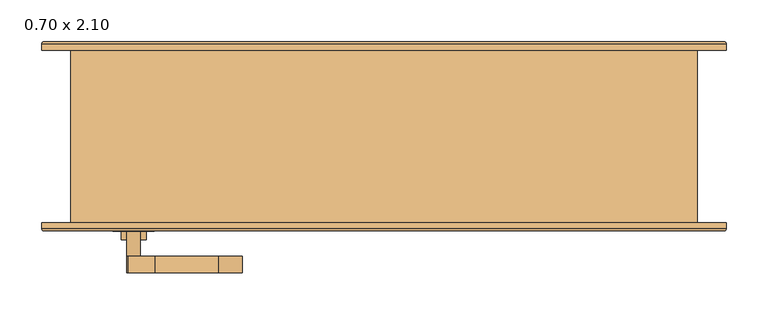
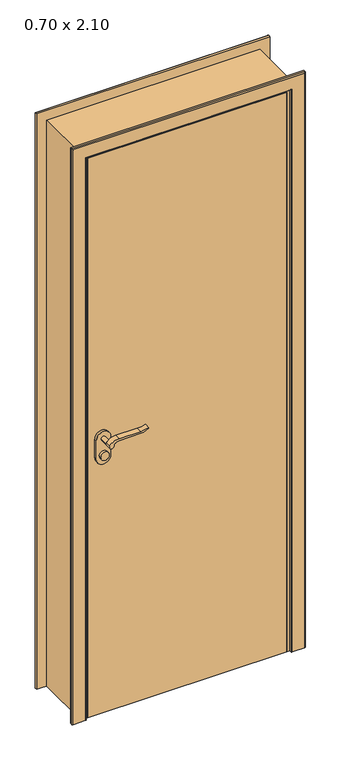
"""IFC4 building model written with IfcOpenShell, lengths in millimetres: door geometry, .CC_ND 300_PORTA SIMPLES DE ABRIR_COM EXTENSÃO : 0.70 x 2.10."""

from ifc_helpers import new_model, si_unit, point, frame, frame_2d, origin, origin_with_axes, place, context, project, spatial, polyline, circle_curve, ellipse_curve, trimmed, segment, composite_curve, outline, extrude, faceted_brep, source, transform, mapped, element, save
from ifc_brep_helpers import plane_surface, cylinder_surface, advanced_brep


def door_0_70_x_2_10_2730a6bb(model_context):
    return source(origin(), model_context, "Body", "SolidModel", [
        extrude(outline(composite_curve([segment(trimmed(circle_curve(frame_2d((964.5, -300.0)), 15.0), [point((964.5, -285.0))], [point((964.5, -315.0))], False, "CARTESIAN"), True, "CONTINUOUS"), segment(trimmed(circle_curve(frame_2d((964.5, -300.0)), 15.0), [point((964.5, -315.0))], [point((964.5, -285.0))], False, "CARTESIAN"), True, "CONTINUOUS")], self_intersect=False)), frame((0.0, -120.7, 0.0), z_axis=(0.0, 1.0, 0.0), x_axis=(0.0, 0.0, 1.0)), (0.0, 0.0, 1.0), 10.0),
        extrude(outline(composite_curve([segment(trimmed(circle_curve(frame_2d((964.5, -300.0)), 15.0), [point((964.5, -285.0))], [point((964.5, -315.0))], False, "CARTESIAN"), True, "CONTINUOUS"), segment(trimmed(circle_curve(frame_2d((964.5, -300.0)), 15.0), [point((964.5, -315.0))], [point((964.5, -285.0))], False, "CARTESIAN"), True, "CONTINUOUS")], self_intersect=False)), frame((0.0, -60.7, 0.0), z_axis=(0.0, 1.0, 0.0), x_axis=(0.0, 0.0, 1.0)), (0.0, 0.0, 1.0), 10.0),
        extrude(outline(composite_curve([segment(trimmed(circle_curve(frame_2d((1024.5, -300.0)), 8.0), [point((1029.1523287, -306.5081363))], [point((1024.5, -292.0))], False, "CARTESIAN"), True, "CONTINUOUS"), segment(trimmed(circle_curve(frame_2d((1019.3738613, -274.6138099)), 18.1261387), [point((1024.5, -292.0))], [point((1037.5, -274.6138099))], True, "CARTESIAN"), True, "CONTINUOUS"), segment(polyline([(1037.5, -274.6138099), (1037.5, -198.3564091)]), True, "CONTINUOUS"), segment(trimmed(circle_curve(frame_2d((1096.7709207, -201.9396612)), 59.3791355), [point((1037.5, -198.3564091))], [point((1046.7135558, -170.0))], False, "CARTESIAN"), True, "CONTINUOUS"), segment(polyline([(1046.7135558, -170.0), (1049.5, -170.0)]), True, "CONTINUOUS"), segment(trimmed(circle_curve(frame_2d((1127.7850638, -198.4227909)), 83.2850902), [point((1049.5, -170.0))], [point((1044.5, -198.3564091))], True, "CARTESIAN"), True, "CONTINUOUS"), segment(polyline([(1044.5, -198.3564091), (1044.5, -274.6325667)]), True, "CONTINUOUS"), segment(trimmed(circle_curve(frame_2d((1007.2555521, -276.3324871)), 37.2832219), [point((1044.5, -274.6325667))], [point((1029.1523287, -306.5081363))], False, "CARTESIAN"), True, "CONTINUOUS")], self_intersect=False)), frame((0.0, -160.7, 0.0), z_axis=(0.0, 1.0, 0.0), x_axis=(0.0, 0.0, 1.0)), (0.0, 0.0, 1.0), 20.0),
        extrude(outline(composite_curve([segment(trimmed(circle_curve(frame_2d((1019.3738682, -274.6138122)), 18.1261318), [point((1024.4999903, -292.0))], [point((1037.5, -274.6138122))], True, "CARTESIAN"), True, "CONTINUOUS"), segment(polyline([(1037.5, -274.6138122), (1037.5, -198.3564091)]), True, "CONTINUOUS"), segment(trimmed(circle_curve(frame_2d((1096.7709207, -201.9396612)), 59.3791355), [point((1037.5, -198.3564091))], [point((1046.7135558, -170.0))], False, "CARTESIAN"), True, "CONTINUOUS"), segment(polyline([(1046.7135558, -170.0), (1049.5, -170.0)]), True, "CONTINUOUS"), segment(trimmed(circle_curve(frame_2d((1127.7850638, -198.4227909)), 83.2850902), [point((1049.5, -170.0))], [point((1044.5, -198.3564091))], True, "CARTESIAN"), True, "CONTINUOUS"), segment(polyline([(1044.5, -198.3564091), (1044.5, -274.6325667)]), True, "CONTINUOUS"), segment(trimmed(circle_curve(frame_2d((1007.2555521, -276.3324871)), 37.2832219), [point((1044.5, -274.6325667))], [point((1029.1523287, -306.5081363))], False, "CARTESIAN"), True, "CONTINUOUS"), segment(trimmed(circle_curve(frame_2d((1024.5, -300.0)), 8.0), [point((1029.1523287, -306.5081363))], [point((1024.4999903, -292.0))], False, "CARTESIAN"), True, "CONTINUOUS")], self_intersect=False)), frame((0.0, -30.7, 0.0), z_axis=(0.0, 1.0, 0.0), x_axis=(0.0, 0.0, 1.0)), (0.0, 0.0, 1.0), 20.0),
        extrude(outline(composite_curve([segment(trimmed(circle_curve(frame_2d((1024.5, -300.0)), 8.0), [point((1024.5, -292.0))], [point((1024.5, -308.0))], False, "CARTESIAN"), True, "CONTINUOUS"), segment(trimmed(circle_curve(frame_2d((1024.5, -300.0)), 8.0), [point((1024.5, -308.0))], [point((1024.5, -292.0))], False, "CARTESIAN"), True, "CONTINUOUS")], self_intersect=False)), frame((0.0, -140.7, 0.0), z_axis=(0.0, 1.0, 0.0), x_axis=(0.0, 0.0, 1.0)), (0.0, 0.0, 1.0), 30.0),
        extrude(outline(composite_curve([segment(trimmed(circle_curve(frame_2d((1024.5, -300.0)), 8.0), [point((1024.5, -292.0))], [point((1024.5, -308.0))], False, "CARTESIAN"), True, "CONTINUOUS"), segment(trimmed(circle_curve(frame_2d((1024.5, -300.0)), 8.0), [point((1024.5, -308.0))], [point((1024.5, -292.0))], False, "CARTESIAN"), True, "CONTINUOUS")], self_intersect=False)), frame((0.0, -60.7, 0.0), z_axis=(0.0, 1.0, 0.0), x_axis=(0.0, 0.0, 1.0)), (0.0, 0.0, 1.0), 30.0),
        extrude(outline(composite_curve([segment(trimmed(circle_curve(frame_2d((954.5, -300.0)), 25.0), [point((954.5, -325.0))], [point((954.5, -275.0))], False, "CARTESIAN"), True, "CONTINUOUS"), segment(polyline([(954.5, -275.0), (1024.5, -275.0)]), True, "CONTINUOUS"), segment(trimmed(circle_curve(frame_2d((1024.5, -300.0)), 25.0), [point((1024.5, -275.0))], [point((1024.5, -325.0))], False, "CARTESIAN"), True, "CONTINUOUS"), segment(polyline([(1024.5, -325.0), (954.5, -325.0)]), True, "CONTINUOUS")], self_intersect=False)), frame((0.0, -110.7, 0.0), z_axis=(0.0, 1.0, 0.0), x_axis=(0.0, 0.0, 1.0)), (0.0, 0.0, 1.0), 10.0),
        extrude(outline(composite_curve([segment(trimmed(circle_curve(frame_2d((954.5, -300.0)), 25.0), [point((954.5, -325.0))], [point((954.5, -275.0))], False, "CARTESIAN"), True, "CONTINUOUS"), segment(polyline([(954.5, -275.0), (1024.5, -275.0)]), True, "CONTINUOUS"), segment(trimmed(circle_curve(frame_2d((1024.5, -300.0)), 25.0), [point((1024.5, -275.0))], [point((1024.5, -325.0))], False, "CARTESIAN"), True, "CONTINUOUS"), segment(polyline([(1024.5, -325.0), (954.5, -325.0)]), True, "CONTINUOUS")], self_intersect=False)), frame((0.0, -70.7, 0.0), z_axis=(0.0, 1.0, 0.0), x_axis=(0.0, 0.0, 1.0)), (0.0, 0.0, 1.0), 10.0),
        faceted_brep([(342.0, 106.0, 0.0), (375.0, 106.0, 0.0), (375.0, -100.7, 0.0), (350.0, -100.7, 0.0), (350.0, -70.7, 0.0), (342.0, -70.7, 0.0), (342.0, 106.0, 2067.0), (-342.0, 106.0, 2067.0), (-342.0, 106.0, 0.0), (-375.0, 106.0, 0.0), (-375.0, 106.0, 2100.0), (375.0, 106.0, 2100.0), (375.0, -100.7, 2100.0), (-375.0, -100.7, 2100.0), (-375.0, -100.7, 0.0), (-350.0, -100.7, 0.0), (-350.0, -100.7, 2075.0), (350.0, -100.7, 2075.0), (350.0, -70.7, 2075.0), (-350.0, -70.7, 2075.0), (-350.0, -70.7, 0.0), (-342.0, -70.7, 0.0), (-342.0, -70.7, 2067.0), (342.0, -70.7, 2067.0)], [[[0, 1, 2, 3, 4, 5]], [[1, 0, 6, 7, 8, 9, 10, 11]], [[2, 1, 11, 12]], [[3, 2, 12, 13, 14, 15, 16, 17]], [[4, 3, 17, 18]], [[5, 4, 18, 19, 20, 21, 22, 23]], [[0, 5, 23, 6]], [[7, 22, 21, 8]], [[8, 21, 20, 15, 14, 9]], [[13, 10, 9, 14]], [[19, 16, 15, 20]], [[12, 11, 10, 13]], [[18, 17, 16, 19]], [[6, 23, 22, 7]]]),
        extrude(outline(polyline([(-350.0, -70.7), (350.0, -70.7), (350.0, -100.7), (-350.0, -100.7), (-350.0, -70.7)])), origin_with_axes(), (0.0, 0.0, 1.0), 2075.0),
        advanced_brep(
        [(-410.0, -100.7, 0.0), (-360.0, -100.7, 0.0), (-360.0, -107.7, 0.0), (-363.0, -110.7, 0.0), (-407.0, -110.7, 0.0), (-410.0, -107.7, 0.0), (-410.0, -100.7, 2135.0), (410.0, -100.7, 2135.0), (410.0, -100.7, 0.0), (360.0, -100.7, 0.0), (360.0, -100.7, 2085.0), (-360.0, -100.7, 2085.0), (-360.0, -107.7, 2085.0), (-363.0, -110.7, 2088.0), (363.0, -110.7, 2088.0), (363.0, -110.7, 0.0), (407.0, -110.7, 0.0), (407.0, -110.7, 2132.0), (-407.0, -110.7, 2132.0), (-410.0, -107.7, 2135.0), (410.0, -107.7, 2135.0), (410.0, -107.7, 0.0), (360.0, -107.7, 0.0), (360.0, -107.7, 2085.0)],
        [
            (0, 1),
            (1, 2),
            (2, 3, circle_curve(frame((-363.0, -107.7, 0.0), z_axis=(0.0, 0.0, -1.0), x_axis=(1.0, 0.0, 0.0)), 3.0)),
            (3, 4),
            (4, 5, circle_curve(frame((-407.0, -107.7, 0.0), z_axis=(0.0, 0.0, -1.0), x_axis=(1.0, 0.0, 0.0)), 3.0)),
            (5, 0),
            (0, 6),
            (6, 7),
            (7, 8),
            (8, 9),
            (9, 10),
            (10, 11),
            (11, 1),
            (11, 12),
            (12, 2),
            (12, 13, ellipse_curve(frame((-363.0, -107.7, 2088.0), z_axis=(-0.7071067811865475, 0.0, -0.7071067811865475), x_axis=(0.7071067811865474, 0.0, -0.7071067811865476)), 4.2426407, 3.0)),
            (13, 3),
            (13, 14),
            (14, 15),
            (15, 16),
            (16, 17),
            (17, 18),
            (18, 4),
            (18, 19, ellipse_curve(frame((-407.0, -107.7, 2132.0), z_axis=(-0.7071067811865475, 0.0, -0.7071067811865475), x_axis=(0.7071067811865474, 0.0, -0.7071067811865476)), 4.2426407, 3.0)),
            (19, 5),
            (19, 6),
            (7, 20),
            (20, 21),
            (21, 8),
            (21, 16, circle_curve(frame((407.0, -107.7, 0.0), z_axis=(0.0, 0.0, -1.0), x_axis=(-1.0, 0.0, 0.0)), 3.0)),
            (15, 22, circle_curve(frame((363.0, -107.7, 0.0), z_axis=(0.0, 0.0, -1.0), x_axis=(-1.0, 0.0, 0.0)), 3.0)),
            (22, 9),
            (23, 10),
            (22, 23),
            (14, 23, ellipse_curve(frame((363.0, -107.7, 2088.0), z_axis=(0.7071067811865475, 0.0, -0.7071067811865475), x_axis=(0.7071067811865474, 0.0, 0.7071067811865476)), 4.2426407, 3.0)),
            (20, 17, ellipse_curve(frame((407.0, -107.7, 2132.0), z_axis=(0.7071067811865475, 0.0, -0.7071067811865475), x_axis=(0.7071067811865474, 0.0, 0.7071067811865476)), 4.2426407, 3.0)),
            (23, 12),
            (19, 20),
        ],
        [
            plane_surface(frame((-360.0, -100.7, 0.0), z_axis=(0.0, 0.0, -1.0), x_axis=(0.0, 1.0, 0.0))),
            plane_surface(frame((-410.0, -100.7, 0.0), z_axis=(0.0, 1.0, 0.0), x_axis=(0.0, 0.0, 1.0))),
            plane_surface(frame((-360.0, -100.7, 0.0), z_axis=(1.0, 0.0, 0.0), x_axis=(0.0, 0.0, 1.0))),
            cylinder_surface(frame((-363.0, -107.7, 0.0), z_axis=(0.0, 0.0, -1.0), x_axis=(1.0, 0.0, 0.0)), 3.0),
            plane_surface(frame((-363.0, -110.7, 0.0), z_axis=(0.0, -1.0, 0.0), x_axis=(0.0, 0.0, 1.0))),
            cylinder_surface(frame((-407.0, -107.7, 0.0), z_axis=(0.0, 0.0, -1.0), x_axis=(1.0, 0.0, 0.0)), 3.0),
            plane_surface(frame((-410.0, -107.7, 0.0), z_axis=(-1.0, 0.0, 0.0), x_axis=(0.0, 0.0, 1.0))),
            plane_surface(frame((410.0, -107.7, 2135.0), z_axis=(1.0, 0.0, 0.0), x_axis=(0.0, 0.0, -1.0))),
            plane_surface(frame((360.0, -100.7, 0.0), z_axis=(0.0, 0.0, -1.0), x_axis=(0.0, 1.0, 0.0))),
            plane_surface(frame((360.0, -100.7, 2085.0), z_axis=(-1.0, 0.0, 0.0), x_axis=(0.0, 0.0, -1.0))),
            cylinder_surface(frame((363.0, -107.7, 2085.0), z_axis=(0.0, 0.0, 1.0), x_axis=(-1.0, 0.0, 0.0)), 3.0),
            cylinder_surface(frame((407.0, -107.7, 2085.0), z_axis=(0.0, 0.0, 1.0), x_axis=(-1.0, 0.0, 0.0)), 3.0),
            plane_surface(frame((-360.0, -100.7, 2085.0), z_axis=(0.0, 0.0, -1.0), x_axis=(1.0, 0.0, 0.0))),
            plane_surface(frame((-410.0, -107.7, 2135.0), z_axis=(0.0, 0.0, 1.0), x_axis=(1.0, 0.0, 0.0))),
            cylinder_surface(frame((-360.0, -107.7, 2088.0), z_axis=(-1.0, 0.0, 0.0), x_axis=(0.0, 0.0, -1.0)), 3.0),
            cylinder_surface(frame((-360.0, -107.7, 2132.0), z_axis=(-1.0, 0.0, 0.0), x_axis=(0.0, 0.0, -1.0)), 3.0),
        ],
        [
            (0, [[1, 2, 3, 4, 5, 6]]),
            (1, [[-1, 7, 8, 9, 10, 11, 12, 13]]),
            (2, [[-2, -13, 14, 15]]),
            (3, [[-3, -15, 16, 17]]),
            (4, [[-4, -17, 18, 19, 20, 21, 22, 23]]),
            (5, [[-5, -23, 24, 25]]),
            (6, [[-6, -25, 26, -7]]),
            (7, [[27, 28, 29, -9]]),
            (8, [[-29, 30, -20, 31, 32, -10]]),
            (9, [[33, -11, -32, 34]]),
            (10, [[35, -34, -31, -19]]),
            (11, [[36, -21, -30, -28]]),
            (12, [[-14, -12, -33, 37]]),
            (13, [[-26, 38, -27, -8]]),
            (14, [[-16, -37, -35, -18]]),
            (15, [[-24, -22, -36, -38]]),
        ],
    ),
        advanced_brep(
        [(410.0, 106.0, 0.0), (360.0, 106.0, 0.0), (360.0, 113.0157283, 0.0), (362.9842717, 116.0, 0.0), (407.0342217, 116.0, 0.0), (410.0, 113.0342217, 0.0), (410.0, 106.0, 2135.0), (-410.0, 106.0, 2135.0), (-410.0, 106.0, 0.0), (-360.0, 106.0, 0.0), (-360.0, 106.0, 2085.0), (360.0, 106.0, 2085.0), (360.0, 113.0157283, 2085.0), (362.9842717, 116.0, 2087.9842717), (-362.9842717, 116.0, 2087.9842717), (-362.9842717, 116.0, 0.0), (-407.0342217, 116.0, 0.0), (-407.0342217, 116.0, 2132.0342217), (407.0342217, 116.0, 2132.0342217), (410.0, 113.0342217, 2135.0), (-410.0, 113.0342217, 2135.0), (-410.0, 113.0342217, 0.0), (-360.0, 113.0157283, 0.0), (-360.0, 113.0157283, 2085.0)],
        [
            (0, 1),
            (1, 2),
            (2, 3, circle_curve(frame((362.9842717, 113.0157283, 0.0), z_axis=(0.0, 0.0, -1.0), x_axis=(1.0, 0.0, 0.0)), 2.9842717)),
            (3, 4),
            (4, 5, circle_curve(frame((407.0342217, 113.0342217, 0.0), z_axis=(0.0, 0.0, -1.0), x_axis=(1.0, 0.0, 0.0)), 2.9657783)),
            (5, 0),
            (0, 6),
            (6, 7),
            (7, 8),
            (8, 9),
            (9, 10),
            (10, 11),
            (11, 1),
            (11, 12),
            (12, 2),
            (12, 13, ellipse_curve(frame((362.9842717, 113.0157283, 2087.9842717), z_axis=(0.7071067811865475, 0.0, -0.7071067811865475), x_axis=(-0.7071067811865474, 0.0, -0.7071067811865476)), 4.2203975, 2.9842717)),
            (13, 3),
            (13, 14),
            (14, 15),
            (15, 16),
            (16, 17),
            (17, 18),
            (18, 4),
            (18, 19, ellipse_curve(frame((407.0342217, 113.0342217, 2132.0342217), z_axis=(0.7071067811865475, 0.0, -0.7071067811865475), x_axis=(-0.7071067811865474, 0.0, -0.7071067811865476)), 4.1942438, 2.9657783)),
            (19, 5),
            (19, 6),
            (7, 20),
            (20, 21),
            (21, 8),
            (21, 16, circle_curve(frame((-407.0342217, 113.0342217, 0.0), z_axis=(0.0, 0.0, -1.0), x_axis=(-1.0, 0.0, 0.0)), 2.9657783)),
            (15, 22, circle_curve(frame((-362.9842717, 113.0157283, 0.0), z_axis=(0.0, 0.0, -1.0), x_axis=(-1.0, 0.0, 0.0)), 2.9842717)),
            (22, 9),
            (23, 10),
            (22, 23),
            (14, 23, ellipse_curve(frame((-362.9842717, 113.0157283, 2087.9842717), z_axis=(-0.7071067811865475, 0.0, -0.7071067811865475), x_axis=(-0.7071067811865474, 0.0, 0.7071067811865476)), 4.2203975, 2.9842717)),
            (20, 17, ellipse_curve(frame((-407.0342217, 113.0342217, 2132.0342217), z_axis=(-0.7071067811865475, 0.0, -0.7071067811865475), x_axis=(-0.7071067811865474, 0.0, 0.7071067811865476)), 4.1942438, 2.9657783)),
            (23, 12),
            (19, 20),
        ],
        [
            plane_surface(frame((360.0, 106.0, 0.0), z_axis=(0.0, 0.0, -1.0), x_axis=(0.0, 1.0, 0.0))),
            plane_surface(frame((410.0, 106.0, 0.0), z_axis=(0.0, -1.0, 0.0), x_axis=(0.0, 0.0, 1.0))),
            plane_surface(frame((360.0, 106.0, 0.0), z_axis=(-1.0, 0.0, 0.0), x_axis=(0.0, 0.0, 1.0))),
            cylinder_surface(frame((362.9842717, 113.0157283, 0.0), z_axis=(0.0, 0.0, -1.0), x_axis=(1.0, 0.0, 0.0)), 2.9842717),
            plane_surface(frame((362.9842717, 116.0, 0.0), z_axis=(0.0, 1.0, 0.0), x_axis=(0.0, 0.0, 1.0))),
            cylinder_surface(frame((407.0342217, 113.0342217, 0.0), z_axis=(0.0, 0.0, -1.0), x_axis=(1.0, 0.0, 0.0)), 2.9657783),
            plane_surface(frame((410.0, 113.0342217, 0.0), z_axis=(1.0, 0.0, 0.0), x_axis=(0.0, 0.0, 1.0))),
            plane_surface(frame((-410.0, 113.0342217, 2135.0), z_axis=(-1.0, 0.0, 0.0), x_axis=(0.0, 0.0, -1.0))),
            plane_surface(frame((-360.0, 106.0, 0.0), z_axis=(0.0, 0.0, -1.0), x_axis=(0.0, 1.0, 0.0))),
            plane_surface(frame((-360.0, 106.0, 2085.0), z_axis=(1.0, 0.0, 0.0), x_axis=(0.0, 0.0, -1.0))),
            cylinder_surface(frame((-362.9842717, 113.0157283, 2085.0), z_axis=(0.0, 0.0, 1.0), x_axis=(-1.0, 0.0, 0.0)), 2.9842717),
            cylinder_surface(frame((-407.0342217, 113.0342217, 2085.0), z_axis=(0.0, 0.0, 1.0), x_axis=(-1.0, 0.0, 0.0)), 2.9657783),
            plane_surface(frame((360.0, 106.0, 2085.0), z_axis=(0.0, 0.0, -1.0), x_axis=(-1.0, 0.0, 0.0))),
            plane_surface(frame((410.0, 113.0342217, 2135.0), z_axis=(0.0, 0.0, 1.0), x_axis=(-1.0, 0.0, 0.0))),
            cylinder_surface(frame((360.0, 113.0157283, 2087.9842717), z_axis=(1.0, 0.0, 0.0), x_axis=(0.0, 0.0, 1.0)), 2.9842717),
            cylinder_surface(frame((360.0, 113.0342217, 2132.0342217), z_axis=(1.0, 0.0, 0.0), x_axis=(0.0, 0.0, 1.0)), 2.9657783),
        ],
        [
            (0, [[1, 2, 3, 4, 5, 6]]),
            (1, [[-1, 7, 8, 9, 10, 11, 12, 13]]),
            (2, [[-2, -13, 14, 15]]),
            (3, [[-3, -15, 16, 17]]),
            (4, [[-4, -17, 18, 19, 20, 21, 22, 23]]),
            (5, [[-5, -23, 24, 25]]),
            (6, [[-6, -25, 26, -7]]),
            (7, [[27, 28, 29, -9]]),
            (8, [[-29, 30, -20, 31, 32, -10]]),
            (9, [[33, -11, -32, 34]]),
            (10, [[35, -34, -31, -19]]),
            (11, [[36, -21, -30, -28]]),
            (12, [[-14, -12, -33, 37]]),
            (13, [[-26, 38, -27, -8]]),
            (14, [[-16, -37, -35, -18]]),
            (15, [[-24, -22, -36, -38]]),
        ],
    ),
    ])


if __name__ == "__main__":
    model = new_model("IFC4")
    model_context = context("Model", 3, world=origin())
    ifc_project = project(units=[si_unit("LENGTHUNIT", "METRE", prefix="MILLI")], contexts=[model_context])
    site = spatial("IfcSite", under=ifc_project)
    building = spatial("IfcBuilding", under=site)
    placement = place(None, origin())
    door_0_70_x_2_10_shape = door_0_70_x_2_10_2730a6bb(model_context)
    element("IfcDoor", 1, ObjectType=".CC_ND 300_PORTA SIMPLES DE ABRIR_COM EXTENSÃO : 0.70 x 2.10", at=placement, inside=building, context=model_context, shape_type="MappedRepresentation", body=[
        mapped(door_0_70_x_2_10_shape, transform((0.0, 0.0, 0.0), x_axis=(1.0, 0.0, 0.0), y_axis=(0.0, 1.0, 0.0), z_axis=(0.0, 0.0, 1.0))),
    ])
    save(model, "model.ifc")

# Revit data of these elements
# Type ".CC_ND 300_PORTA SIMPLES DE ABRIR_COM EXTENSÃO : 0.70 x 2.10"
#   Type Mark = "155"
#   Analytic Construction = "<None>"
#   Rough Width = 0.75 m
#   Espessura moldura externa = 0.01 m
#   Espessura moldura interna = 0.01 m
#   Largura moldura = 0.05 m
#   Extensão acabamento exterior [instance default] = 0.00 m
#   Extensão acabamento interior [instance default] = 0.00 m
#   Espessura batente = 0.025 m
#   Thickness = 0.03 m
#   Altura batente = 2.085 m
#   Aux Arco [instance default] = 0.70 m
#   Rough Height = 2.125 m
#   Height = 2.10 m
#   Width = 0.70 m
#   Moldura interna [instance default] = yes
#   Moldura externa [instance default] = yes
#   Porta = .MADEIRA COM PINTURA ESMALTE BRANCO ACETINADO
#   Moldura = .MADEIRA COM PINTURA ESMALTE BRANCO ACETINADO
#   Maçaneta = .ALUMÍNIO
#   Batente = .MADEIRA COM PINTURA ESMALTE BRANCO ACETINADO
#   Function = (empty or 0)
#   Wall Closure = (empty or 0)
# Element 1 (IfcDoor, ".CC_ND 300_PORTA SIMPLES DE ABRIR_COM EXTENSÃO : 0.70 x 2.10")
#   Extensão acabamento exterior = 0.031 m
#   Extensão acabamento interior = 0.0257 m
#   Aux Arco = 0.7257 m
#   Materials on its faces: ".MADEIRA COM PINTURA ESMALTE BRANCO ACETINADO", ".ALUMÍNIO"
# Materials
#   ".MADEIRA COM PINTURA ESMALTE BRANCO ACETINADO": class ".CC_MADEIRAS", colour RGB 240 240 240, transparency 0, Description = "Madeira com pintura esmalte branco acetinado.", Cost = 0
#   ".ALUMÍNIO": class "CC_METAIS", colour RGB 244 244 244, transparency 0, Description = "Material alumínio", Cost = 0
